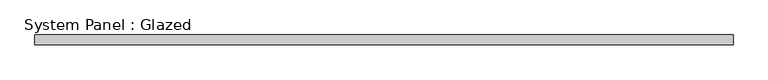
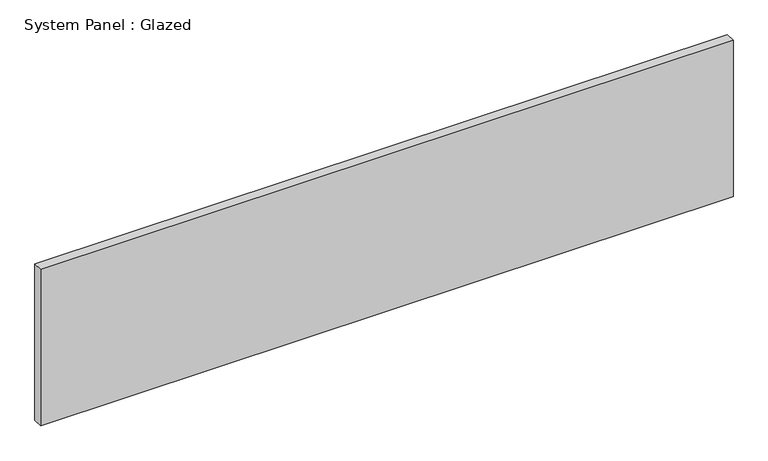
"""IFC4 building model written with IfcOpenShell, lengths in millimetres: plate geometry, System Panel : Glazed."""

from ifc_helpers import new_model, si_unit, origin, origin_with_axes, place, context, project, spatial, polyline, outline, extrude, source, transform, mapped, element, save


def system_panel_glazed_68b51738(model_context):
    return source(origin(), model_context, "Body", "SweptSolid", [
        extrude(outline(polyline([(890.0, 24.5), (-890.0, 24.5), (-890.0, 49.5), (890.0, 49.5), (890.0, 24.5)])), origin_with_axes(), (0.0, 0.0, 1.0), 425.0),
    ])


if __name__ == "__main__":
    model = new_model("IFC4")
    model_context = context("Model", 3, world=origin())
    ifc_project = project(units=[si_unit("LENGTHUNIT", "METRE", prefix="MILLI")], contexts=[model_context])
    site = spatial("IfcSite", under=ifc_project)
    building = spatial("IfcBuilding", under=site)
    placement = place(None, origin())
    system_panel_glazed_shape = system_panel_glazed_68b51738(model_context)
    element("IfcPlate", 1, ObjectType="System Panel : Glazed", at=placement, inside=building, context=model_context, shape_type="MappedRepresentation", body=[
        mapped(system_panel_glazed_shape, transform((0.0, 0.0, 0.0), x_axis=(1.0, 0.0, 0.0), y_axis=(0.0, 1.0, 0.0), z_axis=(0.0, 0.0, 1.0))),
    ])
    save(model, "model.ifc")

# Revit data of these elements
# Type "System Panel : Glazed"
#   Keynote = "H11"
#   Construction Type Id = "GSP4R"
#   Analytic Construction = "1/8 in Pilkington single glazing"
#   Visual Light Transmittance = 0.9
#   Solar Heat Gain Coefficient = 0.86
#   Heat Transfer Coefficient (U) = 6.7069 W/(m²·K)
# Element 1 (IfcPlate, "System Panel : Glazed")
#   Materials on its faces: "Glass"
# Materials
#   "Glass": class "Glass", colour RGB 0 128 192, transparency 0.9, Description = "Soda Lime Glass", Cost = 0
